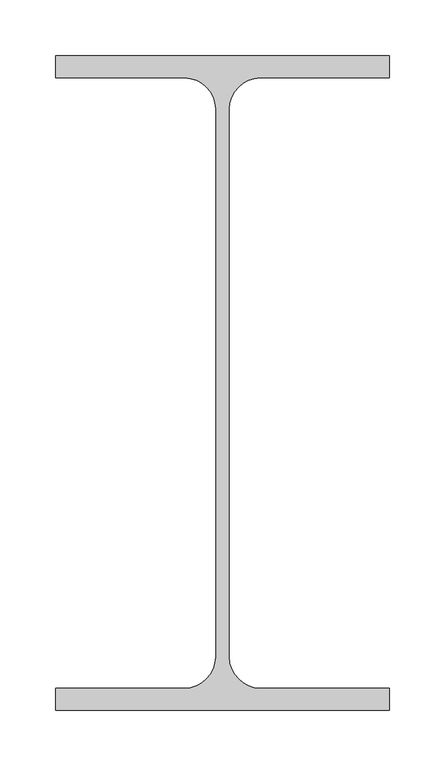
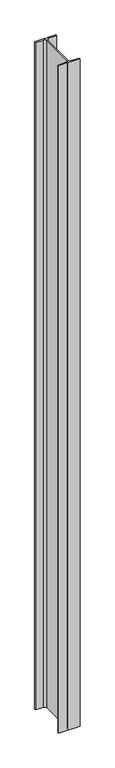
"""IFC4 building model written with IfcOpenShell, lengths in millimetres: column geometry, Steel Column_H_KS : H_SC_AR_S01_H-588x300x12x20_SC1."""

from ifc_helpers import new_model, si_unit, point, frame, frame_2d, origin, place, context, project, spatial, polyline, circle_curve, trimmed, segment, composite_curve, outline, extrude, source, transform, mapped, element, save


def column_e72d12ed(model_context):
    return source(origin(), model_context, "Body", "SweptSolid", [
        extrude(outline(composite_curve([segment(polyline([(150.0, 294.0), (150.0, 274.0), (34.0, 274.0)]), True, "CONTINUOUS"), segment(trimmed(circle_curve(frame_2d((34.0, 246.0)), 28.0), [point((34.0, 274.0))], [point((6.0, 246.0))], True, "CARTESIAN"), True, "CONTINUOUS"), segment(polyline([(6.0, 246.0), (6.0, -246.0)]), True, "CONTINUOUS"), segment(trimmed(circle_curve(frame_2d((34.0, -246.0)), 28.0), [point((6.0, -246.0))], [point((34.0, -274.0))], True, "CARTESIAN"), True, "CONTINUOUS"), segment(polyline([(34.0, -274.0), (150.0, -274.0), (150.0, -294.0), (-150.0, -294.0), (-150.0, -274.0), (-34.0, -274.0)]), True, "CONTINUOUS"), segment(trimmed(circle_curve(frame_2d((-34.0, -246.0)), 28.0), [point((-34.0, -274.0))], [point((-6.0, -246.0))], True, "CARTESIAN"), True, "CONTINUOUS"), segment(polyline([(-6.0, -246.0), (-6.0, 246.0)]), True, "CONTINUOUS"), segment(trimmed(circle_curve(frame_2d((-34.0, 246.0)), 28.0), [point((-6.0, 246.0))], [point((-34.0, 274.0))], True, "CARTESIAN"), True, "CONTINUOUS"), segment(polyline([(-34.0, 274.0), (-150.0, 274.0), (-150.0, 294.0), (150.0, 294.0)]), True, "CONTINUOUS")], self_intersect=False)), frame((0.0, 0.0, 249.9618634), z_axis=(0.0, 0.0, 1.0), x_axis=(1.0, 0.0, 0.0)), (0.0, 0.0, 1.0), 9950.0),
    ])


if __name__ == "__main__":
    model = new_model("IFC4")
    model_context = context("Model", 3, world=origin())
    ifc_project = project(units=[si_unit("LENGTHUNIT", "METRE", prefix="MILLI")], contexts=[model_context])
    site = spatial("IfcSite", under=ifc_project)
    building = spatial("IfcBuilding", under=site)
    placement = place(None, origin())
    column_shape = column_e72d12ed(model_context)
    element("IfcColumn", 1, ObjectType="Steel Column_H_KS : H_SC_AR_S01_H-588x300x12x20_SC1", at=placement, inside=building, context=model_context, shape_type="MappedRepresentation", body=[
        mapped(column_shape, transform((0.0, 0.0, 0.0), x_axis=(1.0, 0.0, 0.0), y_axis=(0.0, 1.0, 0.0), z_axis=(0.0, 0.0, 1.0))),
    ])
    save(model, "model.ifc")

# Revit data of these elements
# Type "Steel Column_H_KS : H_SC_AR_S01_H-588x300x12x20_SC1"
#   Type Comments = "MAIN"
#   Type Mark = "SC1"
#   H_SectionID = "H-588x300x12x20"
#   H_Ratio for Additional Steel Plate = 0.2
#   Width = 30.0 cm
#   Web Thickness = 1.2 cm
#   Web Fillet = 2.8 cm
#   Warping Constant = 7259040.0 cm⁶
#   Torsional Moment of Inertia = 192.717 cm⁴
#   Section Area = 192.5 cm²
#   Plastic Modulus weak axis = 928.0 cm³
#   Plastic Modulus strong axis = 4490.0 cm³
#   Perimeter = 2.30393 m²/m
#   Nominal Weight = 151.00 kgf/m
#   Moment of Inertia weak axis = 9020.00 cm⁴
#   Moment of Inertia strong axis = 118000.00 cm⁴
#   Height = 58.8 cm
#   Flange Thickness = 2.0 cm
#   Elastic Modulus weak axis = 601.0 cm³
#   Elastic Modulus strong axis = 4020.0 cm³
#   Centroid Vertical = 29.4 cm
#   Centroid Horizontal = 15.0 cm
#   Structural Material [instance default] = Steel, 45-345
#   Section Name Key = ""
#   Bolt Spacing = 0
#   Assembly Code = ""
# Element 1 (IfcColumn, "Steel Column_H_KS : H_SC_AR_S01_H-588x300x12x20_SC1")
#   Materials on its faces: "Steel, 45-345"
# Materials
#   "Steel, 45-345": class "Metal", colour RGB 189 187 185, transparency 0, Description = "Steel 345 MPa", Cost = 0
